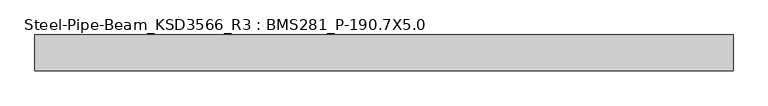
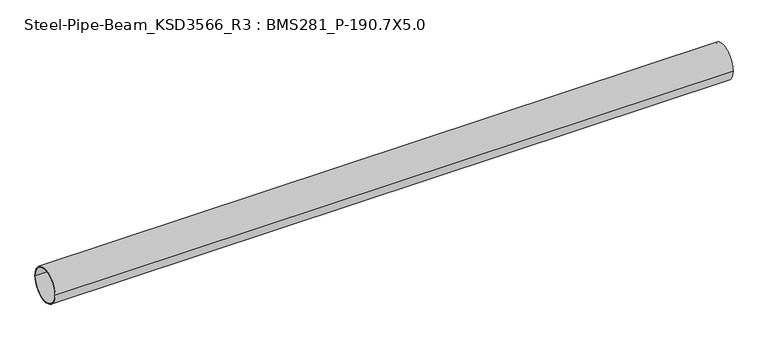
"""IFC4 building model written with IfcOpenShell, lengths in millimetres: member geometry, Steel-Pipe-Beam_KSD3566_R3 : BMS281_P-190.7X5.0."""

from ifc_helpers import new_model, si_unit, point, frame, origin, origin_2d, place, context, project, spatial, circle_curve, trimmed, segment, composite_curve, outline, extrude, source, transform, mapped, element, save


def steel_pipe_beam_ksd3566_r3_bms281_p_190_7x5_0_1667adfa(model_context):
    return source(origin(), model_context, "Body", "SweptSolid", [
        extrude(outline(composite_curve([segment(trimmed(circle_curve(origin_2d(), 95.35), [point((-95.35, 0.0))], [point((95.35, 0.0))], False, "CARTESIAN"), True, "CONTINUOUS"), segment(trimmed(circle_curve(origin_2d(), 95.35), [point((95.35, 0.0))], [point((-95.35, 0.0))], False, "CARTESIAN"), True, "CONTINUOUS")], self_intersect=False), holes=[composite_curve([segment(trimmed(circle_curve(origin_2d(), 90.35), [point((90.35, 0.0))], [point((-90.35, 0.0))], True, "CARTESIAN"), True, "CONTINUOUS"), segment(trimmed(circle_curve(origin_2d(), 90.35), [point((-90.35, 0.0))], [point((90.35, 0.0))], True, "CARTESIAN"), True, "CONTINUOUS")], self_intersect=False)]), frame((-1887.8699719, 0.0, 0.0), z_axis=(1.0, 0.0, 0.0), x_axis=(0.0, 1.0, 0.0)), (0.0, 0.0, 1.0), 3728.144755),
    ])


if __name__ == "__main__":
    model = new_model("IFC4")
    model_context = context("Model", 3, world=origin())
    ifc_project = project(units=[si_unit("LENGTHUNIT", "METRE", prefix="MILLI")], contexts=[model_context])
    site = spatial("IfcSite", under=ifc_project)
    building = spatial("IfcBuilding", under=site)
    placement = place(None, origin())
    steel_pipe_beam_ksd3566_r3_bms281_p_190_7x5_0_shape = steel_pipe_beam_ksd3566_r3_bms281_p_190_7x5_0_1667adfa(model_context)
    element("IfcMember", 1, ObjectType="Steel-Pipe-Beam_KSD3566_R3 : BMS281_P-190.7X5.0", at=placement, inside=building, context=model_context, shape_type="MappedRepresentation", body=[
        mapped(steel_pipe_beam_ksd3566_r3_bms281_p_190_7x5_0_shape, transform((0.0, 0.0, 0.0), x_axis=(1.0, 0.0, 0.0), y_axis=(0.0, 1.0, 0.0), z_axis=(0.0, 0.0, 1.0))),
    ])
    save(model, "model.ifc")

# Revit data of these elements
# Type "Steel-Pipe-Beam_KSD3566_R3 : BMS281_P-190.7X5.0"
#   Keynote = "P-190.7X5.0"
#   SteelWeight = "Light"
#   t = 0.0050 m
#   Surface Area = 0.599102 m²/m
#   Section Area = 29.1697 cm²
#   Mass per Unit Length = 22.8982 kg/m
#   Length [instance default] = 1.5000 m
#   D = 0.1907 m
#   hec_material4 [instance default] = none
#   hec_material3 [instance default] = none
#   hec_material2 [instance default] = none
#   hec_material1 [instance default] = none
#   Structural Material [instance default] = Steel, 45-345
#   Assembly Code = ""
# Element 1 (IfcMember, "Steel-Pipe-Beam_KSD3566_R3 : BMS281_P-190.7X5.0")
#   Structural Material = none
# Materials
#   "Steel, 45-345": class "Metal", colour RGB 189 187 185, transparency 0, Description = "Steel 345 MPa", Cost = 0
